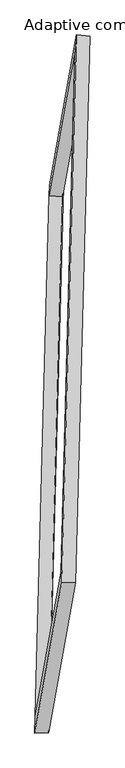
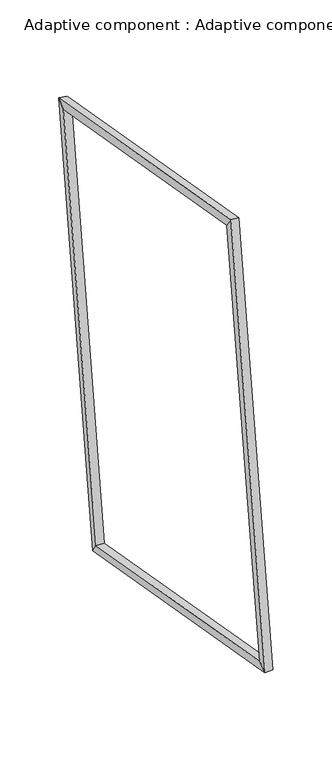
"""IFC4 building model written with IfcOpenShell, lengths in millimetres: proxy geometry, Adaptive component : Adaptive component."""

from ifc_helpers import new_model, si_unit, origin, place, context, project, spatial, faceted_brep, source, transform, mapped, element, save


def adaptive_component_adaptive_component_f4321cc7(model_context):
    return source(origin(), model_context, "Body", "Brep", [
        faceted_brep([(69.3870737, 1125.967215, 2751.2334198), (134.0411515, 1120.0158007, 2746.7674922), (69.509618, -1292.7347073, 3239.3162643), (4.6856571, -1293.1350043, 3245.0788563), (76.6518956, 1202.3631798, 2801.7345616), (8.5491649, -1343.9097716, 3321.5411523), (141.3059733, 1196.4117655, 2797.268634), (73.3731257, -1343.5094746, 3315.7785603), (-51.0628007, -1962.6310953, -57.9685235), (-116.1190009, -1964.3217063, -58.5569622), (-116.9052704, -2040.9304826, -109.2517704), (-51.8490702, -2039.2398716, -108.6633316), (13.4687327, 450.1194126, -550.5172957), (-51.4175843, 454.780513, -552.4023988), (-48.8025397, 505.3424688, -629.0583611), (16.0837773, 500.6813684, -627.173258)], [[[0, 1, 2, 3]], [[4, 0, 3, 5]], [[6, 4, 5, 7]], [[1, 6, 7, 2]], [[3, 2, 8, 9]], [[5, 3, 9, 10]], [[7, 5, 10, 11]], [[2, 7, 11, 8]], [[9, 8, 12, 13]], [[10, 9, 13, 14]], [[11, 10, 14, 15]], [[8, 11, 15, 12]], [[13, 12, 1, 0]], [[14, 13, 0, 4]], [[15, 14, 4, 6]], [[12, 15, 6, 1]]]),
    ])


if __name__ == "__main__":
    model = new_model("IFC4")
    model_context = context("Model", 3, world=origin())
    ifc_project = project(units=[si_unit("LENGTHUNIT", "METRE", prefix="MILLI")], contexts=[model_context])
    site = spatial("IfcSite", under=ifc_project)
    building = spatial("IfcBuilding", under=site)
    placement = place(None, origin())
    adaptive_component_adaptive_component_shape = adaptive_component_adaptive_component_f4321cc7(model_context)
    element("IfcBuildingElementProxy", 1, Name="Adaptive component : Adaptive component", ObjectType="Adaptive component : Adaptive component", at=placement, inside=building, context=model_context, shape_type="MappedRepresentation", body=[
        mapped(adaptive_component_adaptive_component_shape, transform((0.0, 0.0, 0.0), x_axis=(1.0, 0.0, 0.0), y_axis=(0.0, 1.0, 0.0), z_axis=(0.0, 0.0, 1.0))),
    ])
    save(model, "model.ifc")

# Revit data of these elements
# Type "Adaptive component : Adaptive component"
#   r [instance default] = 2063.125 mm
#   2r [instance default] = 4126.251 mm
#   Number [instance default] = 5
#   Default Elevation = 0
# Element 1 (IfcBuildingElementProxy, "Adaptive component : Adaptive component")
#   r = 2178.995 mm
#   2r = 4357.99 mm
#   Number = 9
